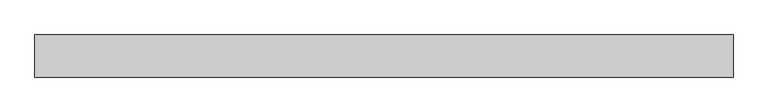
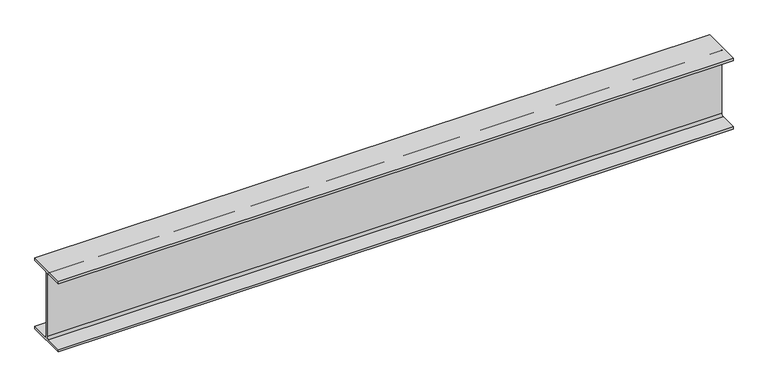
"""IFC4 building model written with IfcOpenShell, lengths in millimetres: beam geometry, Old_Steel Beam_H-KSD3502 : H_SB_ASB_H-200×200x8x12."""

from ifc_helpers import new_model, si_unit, point, frame, frame_2d, origin, place, context, project, spatial, polyline, circle_curve, trimmed, segment, composite_curve, outline, extrude, source, transform, mapped, element, save


def beam_0adccc4e(model_context):
    return source(origin(), model_context, "Body", "SweptSolid", [
        extrude(outline(composite_curve([segment(polyline([(82.5, -141.5), (82.5, -151.7), (-82.5, -151.7), (-82.5, -141.5), (-11.9, -141.5)]), True, "CONTINUOUS"), segment(trimmed(circle_curve(frame_2d((-11.9, -132.6)), 8.9), [point((-11.9, -141.5))], [point((-3.0, -132.6))], True, "CARTESIAN"), True, "CONTINUOUS"), segment(polyline([(-3.0, -132.6), (-3.0, 132.6)]), True, "CONTINUOUS"), segment(trimmed(circle_curve(frame_2d((-11.9, 132.6)), 8.9), [point((-3.0, 132.6))], [point((-11.9, 141.5))], True, "CARTESIAN"), True, "CONTINUOUS"), segment(polyline([(-11.9, 141.5), (-82.5, 141.5), (-82.5, 151.7), (82.5, 151.7), (82.5, 141.5), (11.9, 141.5)]), True, "CONTINUOUS"), segment(trimmed(circle_curve(frame_2d((11.9, 132.6)), 8.9), [point((11.9, 141.5))], [point((3.0, 132.6))], True, "CARTESIAN"), True, "CONTINUOUS"), segment(polyline([(3.0, 132.6), (3.0, -132.6)]), True, "CONTINUOUS"), segment(trimmed(circle_curve(frame_2d((11.9, -132.6)), 8.9), [point((3.0, -132.6))], [point((11.9, -141.5))], True, "CARTESIAN"), True, "CONTINUOUS"), segment(polyline([(11.9, -141.5), (82.5, -141.5)]), True, "CONTINUOUS")], self_intersect=False)), frame((-1342.1060823, 0.0, 0.0), z_axis=(1.0, 0.0, 0.0), x_axis=(0.0, 1.0, 0.0)), (0.0, 0.0, 1.0), 2735.8528348),
    ])


if __name__ == "__main__":
    model = new_model("IFC4")
    model_context = context("Model", 3, world=origin())
    ifc_project = project(units=[si_unit("LENGTHUNIT", "METRE", prefix="MILLI")], contexts=[model_context])
    site = spatial("IfcSite", under=ifc_project)
    building = spatial("IfcBuilding", under=site)
    placement = place(None, origin())
    beam_shape = beam_0adccc4e(model_context)
    element("IfcBeam", 1, ObjectType="Old_Steel Beam_H-KSD3502 : H_SB_ASB_H-200×200x8x12", at=placement, inside=building, context=model_context, shape_type="MappedRepresentation", body=[
        mapped(beam_shape, transform((0.0, 0.0, 0.0), x_axis=(1.0, 0.0, 0.0), y_axis=(0.0, 1.0, 0.0), z_axis=(0.0, 0.0, 1.0))),
    ])
    save(model, "model.ifc")

# Revit data of these elements
# Type "Old_Steel Beam_H-KSD3502 : H_SB_ASB_H-200×200x8x12"
#   Width = 20.0 cm
#   Web Thickness = 0.8 cm
#   Web Fillet = 1.3 cm
#   Warping Constant = 141376.0 cm⁶
#   Torsional Moment of Inertia = 26.2485 cm⁴
#   Torsional Modulus = 1.0 cm³
#   Section Area = 63.53 cm²
#   Plastic Modulus weak axis = 244.0 cm³
#   Plastic Modulus strong axis = 525.0 cm³
#   Perimeter = 1.16 m²/m
#   Nominal Weight = 49.90 kgf/m
#   Moment of Inertia weak axis = 1600.00 cm⁴
#   Moment of Inertia strong axis = 4720.00 cm⁴
#   Height = 20.0 cm
#   Flange Thickness = 1.2 cm
#   Elastic Modulus weak axis = 160.0 cm³
#   Elastic Modulus strong axis = 472.0 cm³
#   Centroid Vertical = 10.0 cm
#   Centroid Horizontal = 10.0 cm
#   Length [instance default] = 1.5240 m
#   Structural Material [instance default] = Steel, 45-345
#   Assembly Code = ""
# Element 1 (IfcBeam, "Old_Steel Beam_H-KSD3502 : H_SB_ASB_H-200×200x8x12")
#   Structural Material = none
# Materials
#   "Steel, 45-345": class "Metal", colour RGB 189 187 185, transparency 0, Description = "Steel 345 MPa", Cost = 0
